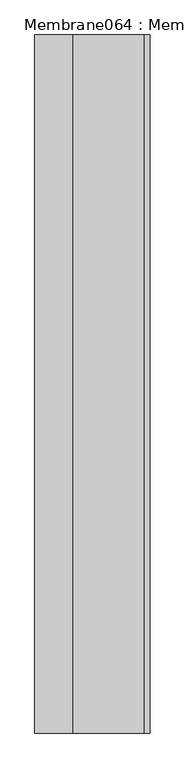
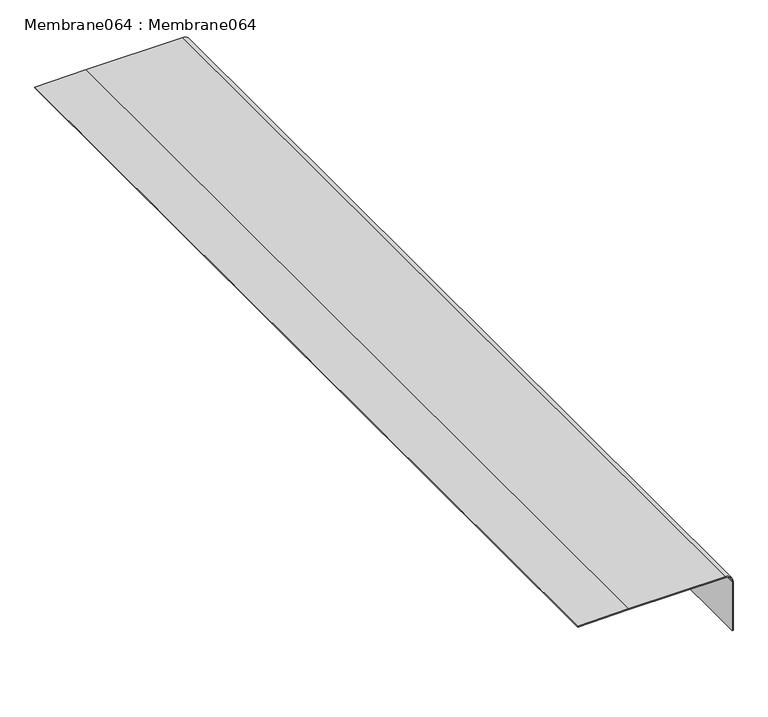
"""IFC4 building model written with IfcOpenShell, lengths in millimetres: proxy geometry, Membrane064 : Membrane064."""

from ifc_helpers import new_model, si_unit, point, frame, frame_2d, origin, place, context, project, spatial, polyline, circle_curve, trimmed, segment, composite_curve, outline, extrude, source, transform, mapped, element, save


def membrane064_membrane064_39c6496e(model_context):
    return source(origin(), model_context, "Body", "SweptSolid", [
        extrude(outline(composite_curve([segment(polyline([(40234.8417335, -4371.0279678), (40125.2457074, -4371.0279678), (40125.2457074, -4369.0279678), (40234.8417335, -4369.0279678)]), True, "CONTINUOUS"), segment(trimmed(circle_curve(frame_2d((40234.8417335, -4386.0279678)), 17.0), [point((40234.8417335, -4369.0279678))], [point((40251.8417335, -4386.0279678))], False, "CARTESIAN"), True, "CONTINUOUS"), segment(polyline([(40251.8417335, -4386.0279678), (40251.8417335, -4591.7190058), (40250.2861996, -4699.8063764), (40248.2859925, -4699.8063764), (40249.8417335, -4591.7046151), (40249.8417335, -4386.0279678)]), True, "CONTINUOUS"), segment(trimmed(circle_curve(frame_2d((40234.8417335, -4386.0279678)), 15.0), [point((40249.8417335, -4386.0279678))], [point((40234.8417335, -4371.0279678))], True, "CARTESIAN"), True, "CONTINUOUS")], self_intersect=False)), frame((0.0, -1052.8906574, 0.0), z_axis=(0.0, 1.0, 0.0), x_axis=(0.0, 0.0, 1.0)), (0.0, 0.0, 1.0), 2000.0),
    ])


if __name__ == "__main__":
    model = new_model("IFC4")
    model_context = context("Model", 3, world=origin())
    ifc_project = project(units=[si_unit("LENGTHUNIT", "METRE", prefix="MILLI")], contexts=[model_context])
    site = spatial("IfcSite", under=ifc_project)
    building = spatial("IfcBuilding", under=site)
    placement = place(None, origin())
    membrane064_membrane064_shape = membrane064_membrane064_39c6496e(model_context)
    element("IfcBuildingElementProxy", 1, Name="Membrane064 : Membrane064", ObjectType="Membrane064 : Membrane064", at=placement, inside=building, context=model_context, shape_type="MappedRepresentation", body=[
        mapped(membrane064_membrane064_shape, transform((0.0, 0.0, 0.0), x_axis=(1.0, 0.0, 0.0), y_axis=(0.0, 1.0, 0.0), z_axis=(0.0, 0.0, 1.0))),
    ])
    save(model, "model.ifc")

# Revit data of these elements
# Type "Membrane064 : Membrane064"
#   NameOverride = "Membrane064"
# Element 1 (IfcBuildingElementProxy, "Membrane064 : Membrane064")
#   Materials on its faces: "THREE PLY BUILT UP ROOF MEMBRANE"
# Materials
#   "THREE PLY BUILT UP ROOF MEMBRANE": class "Unassigned", colour RGB 63 63 63, transparency 0
